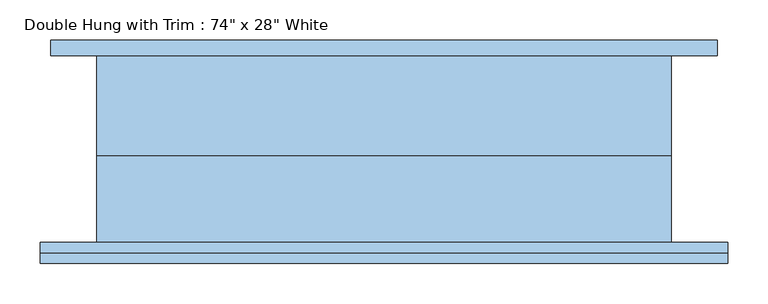
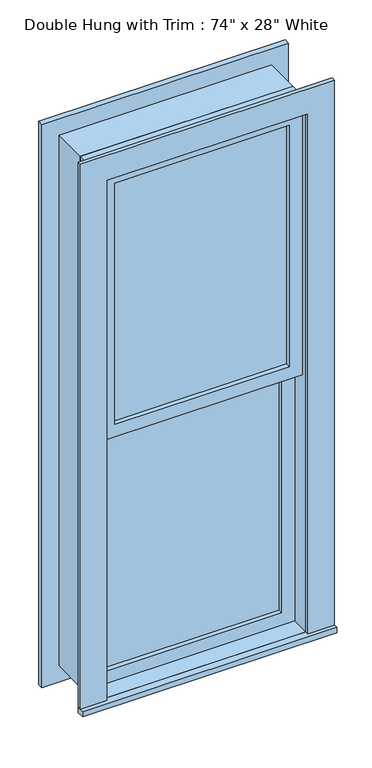
"""IFC4 building model written with IfcOpenShell, lengths in millimetres: window geometry."""

from ifc_helpers import new_model, si_unit, frame, origin, place, context, project, spatial, polyline, outline, extrude, source, transform, mapped, element, save


def window_ba152081(model_context):
    return source(origin(), model_context, "Body", "SweptSolid", [
        extrude(outline(polyline([(-292.1, -36.5125008), (-292.1, -23.8125008), (292.1, -23.8125008), (292.1, -36.5125008), (-292.1, -36.5125008)])), frame((0.0, 0.0, 571.5), z_axis=(0.0, 0.0, 1.0), x_axis=(1.0, 0.0, 0.0)), (0.0, 0.0, 1.0), 854.075),
        extrude(outline(polyline([(1470.025, -336.55), (527.05, -336.55), (527.05, 336.55), (1470.025, 336.55), (1470.025, -336.55)]), holes=[polyline([(1425.575, -292.1), (1425.575, 292.1), (571.5, 292.1), (571.5, -292.1), (1425.575, -292.1)])]), frame((0.0, -52.3875008, 0.0), z_axis=(0.0, 1.0, 0.0), x_axis=(0.0, 0.0, 1.0)), (0.0, 0.0, 1.0), 44.45),
        extrude(outline(polyline([(-425.45, -141.2875008), (-425.45, -115.8875008), (425.45, -115.8875008), (425.45, -141.2875008), (-425.45, -141.2875008)])), frame((0.0, 0.0, 508.0), z_axis=(0.0, 0.0, 1.0), x_axis=(1.0, 0.0, 0.0)), (0.0, 0.0, 1.0), 19.05),
        extrude(outline(polyline([(2368.55, -336.55), (2368.55, 336.55), (527.05, 336.55), (527.05, 425.45), (2457.45, 425.45), (2457.45, -425.45), (527.05, -425.45), (527.05, -336.55), (2368.55, -336.55)])), frame((0.0, -128.5875008, 0.0), z_axis=(0.0, 1.0, 0.0), x_axis=(0.0, 0.0, 1.0)), (0.0, 0.0, 1.0), 12.7),
        extrude(outline(polyline([(2444.75, 412.75), (2444.75, -412.75), (450.85, -412.75), (450.85, 412.75), (2444.75, 412.75)]), holes=[polyline([(2355.85, 323.85), (539.75, 323.85), (539.75, -323.85), (2355.85, -323.85), (2355.85, 323.85)])]), frame((0.0, 115.8875008, 0.0), z_axis=(0.0, 1.0, 0.0), x_axis=(0.0, 0.0, 1.0)), (0.0, 0.0, 1.0), 19.05),
        extrude(outline(polyline([(292.1, -68.2625008), (292.1, -80.9625008), (-292.1, -80.9625008), (-292.1, -68.2625008), (292.1, -68.2625008)])), frame((0.0, 0.0, 1470.025), z_axis=(0.0, 0.0, 1.0), x_axis=(1.0, 0.0, 0.0)), (0.0, 0.0, 1.0), 854.075),
        extrude(outline(polyline([(2368.55, -336.55), (1425.575, -336.55), (1425.575, 336.55), (2368.55, 336.55), (2368.55, -336.55)]), holes=[polyline([(2324.1, -292.1), (2324.1, 292.1), (1470.025, 292.1), (1470.025, -292.1), (2324.1, -292.1)])]), frame((0.0, -96.8375008, 0.0), z_axis=(0.0, 1.0, 0.0), x_axis=(0.0, 0.0, 1.0)), (0.0, 0.0, 1.0), 44.45),
        extrude(outline(polyline([(2387.6, -355.6), (508.0, -355.6), (508.0, 355.6), (2387.6, 355.6), (2387.6, -355.6)]), holes=[polyline([(2355.85, -323.85), (2355.85, 323.85), (539.75, 323.85), (539.75, -323.85), (2355.85, -323.85)])]), frame((0.0, -7.9375008, 0.0), z_axis=(0.0, 1.0, 0.0), x_axis=(0.0, 0.0, 1.0)), (0.0, 0.0, 1.0), 123.8250015),
        extrude(outline(polyline([(2387.6, 355.6), (2387.6, -355.6), (508.0, -355.6), (508.0, 355.6), (2387.6, 355.6)]), holes=[polyline([(2368.55, 336.55), (527.05, 336.55), (527.05, -336.55), (2368.55, -336.55), (2368.55, 336.55)])]), frame((0.0, -115.8875008, 0.0), z_axis=(0.0, 1.0, 0.0), x_axis=(0.0, 0.0, 1.0)), (0.0, 0.0, 1.0), 107.95),
    ])


if __name__ == "__main__":
    model = new_model("IFC4")
    model_context = context("Model", 3, world=origin())
    ifc_project = project(units=[si_unit("LENGTHUNIT", "METRE", prefix="MILLI")], contexts=[model_context])
    site = spatial("IfcSite", under=ifc_project)
    building = spatial("IfcBuilding", under=site)
    placement = place(None, origin())
    window_shape = window_ba152081(model_context)
    element("IfcWindow", 1, ObjectType="Double Hung with Trim : 74\" x 28\" White", at=placement, inside=building, context=model_context, shape_type="MappedRepresentation", body=[
        mapped(window_shape, transform((0.0, 0.0, 0.0), x_axis=(1.0, 0.0, 0.0), y_axis=(0.0, 1.0, 0.0), z_axis=(0.0, 0.0, 1.0))),
    ])
    save(model, "model.ifc")

# Revit data of these elements
# Type "Double Hung with Trim : 74\" x 28\" White"
#   Type Mark = "78"
#   Construction Type Id = "GSP4R"
#   Assembly Code = "B2020100"
#   Analytic Construction = "1/8 in Pilkington single glazing"
#   Visual Light Transmittance = 0.9
#   Solar Heat Gain Coefficient = 0.78
#   Heat Transfer Coefficient (U) = 3.6886 W/(m²·K)
#   Height = 6' - 2"
#   Default Sill Height = 1' - 8"
#   Trim Projection - Ext. = 0' - 0 1/2"
#   Trim Projection - Int. = 0' - 0 3/4"
#   Trim Width - Exterior = 0' - 3 1/2"
#   Trim Width - Interior = 0' - 3 1/2"
#   Width = 2' - 4"
#   Window Inset = 0' - 0 3/4"
#   COBie.Type = no
#   Glass Pane Material = Glass
#   Sash Material = Sash - White
#   Trim Exterior Material = Trim - White
#   Trim Interior Material = Trim - White
#   Wall Closure = (empty or 0)
# Element 1 (IfcWindow, "Double Hung with Trim : 74\" x 28\" White")
#   Materials on its faces: "Sash - White", "Trim - White", "Glass"
# Materials
#   "Glass": class "Glass", colour RGB 0 128 192, transparency 0.75, Description = "Soda Lime Glass", Cost = 0
#   "Sash - White": class "Wood", colour RGB 255 255 255, transparency 0, Cost = 0
#   "Trim - White": class "Wood", colour RGB 255 255 255, transparency 0, Cost = 0
